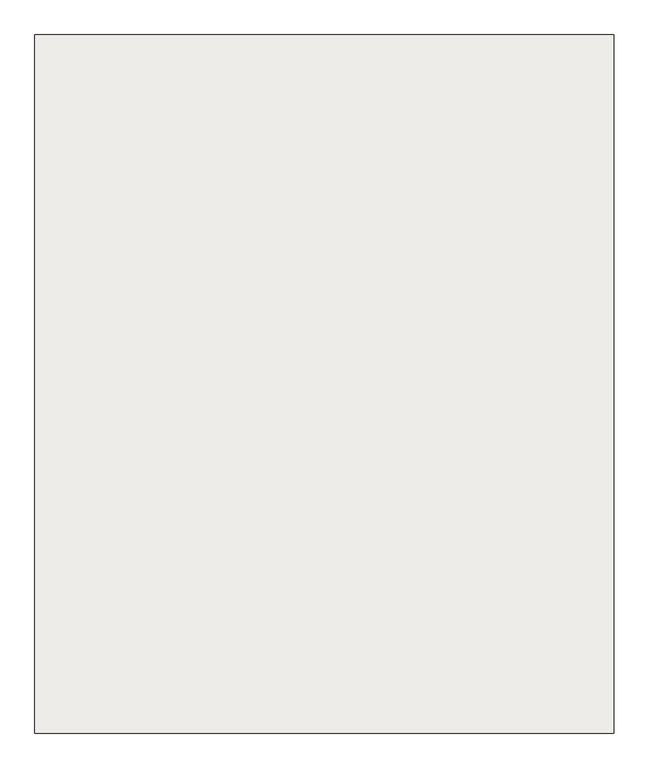
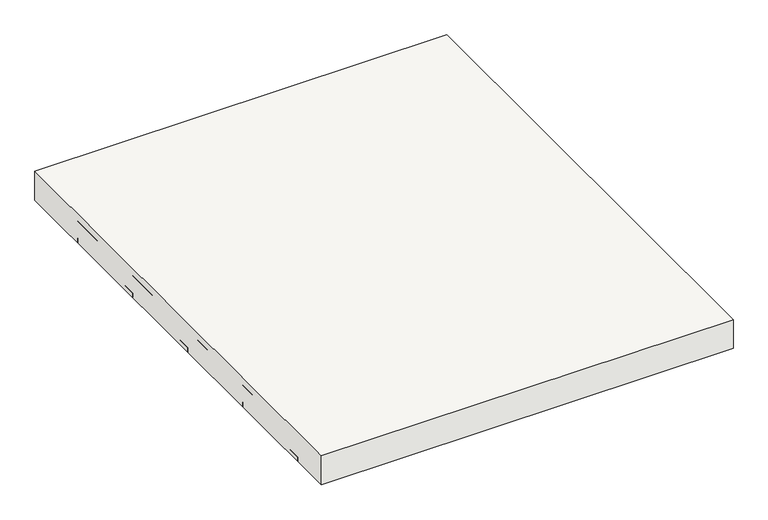
"""IFC4 building model written with IfcOpenShell, lengths in millimetres: slab geometry, Pano 13 (16 cm)."""

import ifcopenshell
import ifcopenshell.guid

model = None  # the IFC model being written
_history = None  # IfcOwnerHistory: only IFC2X3 demands one
_inside = {}  # id of a spatial element -> (the spatial element, [elements in it])
_under = {}  # id of a project, library or spatial element -> (it, [spatial elements below it])
_declared = {}  # id of a project -> (the project, [libraries it declares])
_typed = {}  # id of a type object -> (the type object, [elements of that type])
_made_of = {}  # id of a material, layer set ... -> (it, [elements and type objects made of it])


def new_model(schema):
    """Start an empty IFC model of exactly this schema.

    Asked for "IFC4X3", IfcOpenShell would pick the latest addendum, in which some entities
    have other attributes; the version numbers below select the first issue.
    IFC2X3 requires an IfcOwnerHistory on every rooted entity: one is made here for all.
    """
    global model, _history
    if schema == "IFC4X3":
        model = ifcopenshell.file(schema_version=(4, 3, 0, 0))
    else:
        model = ifcopenshell.file(schema=schema)
    _inside.clear()
    _under.clear()
    _declared.clear()
    _typed.clear()
    _made_of.clear()
    _history = None
    if model.schema == "IFC2X3":
        org = make("IfcOrganization", Name="unknown")
        user = make(
            "IfcPersonAndOrganization",
            ThePerson=make("IfcPerson", FamilyName="unknown"),
            TheOrganization=org,
        )
        app = make(
            "IfcApplication",
            ApplicationDeveloper=org,
            Version="unknown",
            ApplicationFullName="unknown",
            ApplicationIdentifier="unknown",
        )
        _history = make(
            "IfcOwnerHistory",
            OwningUser=user,
            OwningApplication=app,
            ChangeAction="ADDED",
            CreationDate=0,
        )
    return model


def make(cls, **values):
    """One entity of the class cls with the attributes given. An attribute that is None is left unset."""
    return model.create_entity(
        cls, **{name: value for name, value in values.items() if value is not None}
    )


def rooted(cls, **values):
    """An entity with a GlobalId (a new one), such as an element, a storey or a relation."""
    return make(cls, GlobalId=ifcopenshell.guid.new(), OwnerHistory=_history, **values)


def si_unit(unit_type, name, prefix=None):
    """IfcSIUnit, for example si_unit("LENGTHUNIT", "METRE", prefix="MILLI")."""
    return make("IfcSIUnit", UnitType=unit_type, Prefix=prefix, Name=name)


def assignment(units):
    """IfcUnitAssignment: the units of a project."""
    return None if units is None else make("IfcUnitAssignment", Units=units)


def point(xyz):
    """IfcCartesianPoint."""
    return None if xyz is None else make("IfcCartesianPoint", Coordinates=xyz)


def direction(xyz):
    """IfcDirection."""
    return None if xyz is None else make("IfcDirection", DirectionRatios=xyz)


def frame(location, z_axis=None, x_axis=None):
    """IfcAxis2Placement3D, a coordinate frame: its origin and axes. An axis left out is left unset."""
    return make(
        "IfcAxis2Placement3D",
        Location=point(location),
        Axis=direction(z_axis),
        RefDirection=direction(x_axis),
    )


def origin():
    """The frame at (0, 0, 0) with its axes left unset."""
    return frame((0.0, 0.0, 0.0))


def origin_with_axes():
    """The frame at (0, 0, 0) with the z axis (0, 0, 1) and the x axis (1, 0, 0) written out."""
    return frame((0.0, 0.0, 0.0), z_axis=(0.0, 0.0, 1.0), x_axis=(1.0, 0.0, 0.0))


def place(relative_to, where):
    """IfcLocalPlacement: puts the frame where relative to a parent placement (None: the world)."""
    return make(
        "IfcLocalPlacement", PlacementRelTo=relative_to, RelativePlacement=where
    )


def context(
    kind, dimensions, precision=None, world=None, true_north=None, identifier=None
):
    """IfcGeometricRepresentationContext, for example the 3D "Model" context."""
    return make(
        "IfcGeometricRepresentationContext",
        ContextIdentifier=identifier,
        ContextType=kind,
        CoordinateSpaceDimension=dimensions,
        Precision=precision,
        WorldCoordinateSystem=world,
        TrueNorth=true_north,
    )


def project(units=None, contexts=None):
    """IfcProject with its units and contexts."""
    return rooted(
        "IfcProject",
        Name="project",
        RepresentationContexts=contexts,
        UnitsInContext=assignment(units),
    )


def spatial(cls, under=None, at=None, **own):
    """A site, building, storey or space (cls), placed at a placement, below another one or the project."""
    s = rooted(cls, ObjectPlacement=at, **own)
    if under is not None:
        _under.setdefault(under.id(), (under, []))[1].append(s)
    return s


def polyline(points):
    """IfcPolyline through the points."""
    return make("IfcPolyline", Points=[point(p) for p in points])


def outline(outer, holes=None, kind="AREA"):
    """IfcArbitraryClosedProfileDef: a profile drawn as a closed curve; with holes, ...WithVoids."""
    if holes is None:
        return make("IfcArbitraryClosedProfileDef", ProfileType=kind, OuterCurve=outer)
    return make(
        "IfcArbitraryProfileDefWithVoids",
        ProfileType=kind,
        OuterCurve=outer,
        InnerCurves=holes,
    )


def extrude(swept, where, along, depth):
    """IfcExtrudedAreaSolid: the profile swept, set in the frame where, extruded along a direction by depth."""
    return make(
        "IfcExtrudedAreaSolid",
        SweptArea=swept,
        Position=where,
        ExtrudedDirection=direction(along),
        Depth=depth,
    )


def shape(context_of_items, identifier, shape_type, items):
    """IfcShapeRepresentation: the items that make up one representation, for example the "Body"."""
    return make(
        "IfcShapeRepresentation",
        ContextOfItems=context_of_items,
        RepresentationIdentifier=identifier,
        RepresentationType=shape_type,
        Items=items,
    )


def source(mapping_origin, context_of_items, identifier, shape_type, items):
    """IfcRepresentationMap: a shape defined once, which mapped items show again and again."""
    return make(
        "IfcRepresentationMap",
        MappingOrigin=mapping_origin,
        MappedRepresentation=shape(context_of_items, identifier, shape_type, items),
    )


def transform(
    local_origin,
    x_axis=None,
    y_axis=None,
    z_axis=None,
    scale=None,
    scale2=None,
    scale3=None,
    uniform=True,
):
    """IfcCartesianTransformationOperator3D, or its non-uniform kind. x_axis, y_axis, z_axis: its Axis1, 2, 3."""
    if uniform:
        return make(
            "IfcCartesianTransformationOperator3D",
            Axis1=direction(x_axis),
            Axis2=direction(y_axis),
            LocalOrigin=point(local_origin),
            Scale=scale,
            Axis3=direction(z_axis),
        )
    return make(
        "IfcCartesianTransformationOperator3DnonUniform",
        Axis1=direction(x_axis),
        Axis2=direction(y_axis),
        LocalOrigin=point(local_origin),
        Scale=scale,
        Axis3=direction(z_axis),
        Scale2=scale2,
        Scale3=scale3,
    )


def mapped(mapping_source, mapping_target):
    """IfcMappedItem: shows the shape of a source again, moved by a transform."""
    return make(
        "IfcMappedItem", MappingSource=mapping_source, MappingTarget=mapping_target
    )


def made_of(thing, what):
    """Note that an element or type object is made of a material, layer set ...; save() writes the relation."""
    if what is not None:
        _made_of.setdefault(what.id(), (what, []))[1].append(thing)
    return thing


def element(
    cls,
    number,
    at=None,
    inside=None,
    cuts=None,
    type_object=None,
    material=None,
    context=None,
    identifier="Body",
    shape_type=None,
    held_by="IfcProductDefinitionShape",
    body=None,
    shapes=None,
    **own,
):
    """One element of the class cls, such as IfcWall. Its Tag is "e" and its number.

    at: its placement. inside: the storey or other place that contains it. cuts: it is an
    opening in that element (IfcRelVoidsElement). A single representation is given by context,
    identifier, shape_type and body (its items); several are given by shapes. held_by: the class
    of the entity that holds the representations. save() writes the other relations.
    """
    e = rooted(cls, Tag="e%d" % number, ObjectPlacement=at, **own)
    if body is not None:
        shapes = [shape(context, identifier, shape_type, body)]
    if shapes is not None:
        e.Representation = make(held_by, Representations=shapes)
    if inside is not None:
        _inside.setdefault(inside.id(), (inside, []))[1].append(e)
    if cuts is not None:
        rooted(
            "IfcRelVoidsElement", RelatingBuildingElement=cuts, RelatedOpeningElement=e
        )
    if type_object is not None:
        _typed.setdefault(type_object.id(), (type_object, []))[1].append(e)
    return made_of(e, material)


def aggregate(whole, parts):
    """IfcRelAggregates: a whole, such as a stair, and the parts it consists of."""
    return rooted("IfcRelAggregates", RelatingObject=whole, RelatedObjects=parts)


def save(model, path):
    """Write the relations noted so far, then the file.

    IfcRelAggregates (storeys below a building ...), IfcRelContainedInSpatialStructure (elements
    in a storey), IfcRelDefinesByType, IfcRelAssociatesMaterial and IfcRelDeclares: one each for
    every whole, place, type object, material and project.
    """
    for whole, parts in _under.values():
        aggregate(whole, parts)
    for where, things in _inside.values():
        rooted(
            "IfcRelContainedInSpatialStructure",
            RelatedElements=things,
            RelatingStructure=where,
        )
    for kind, things in _typed.values():
        rooted("IfcRelDefinesByType", RelatedObjects=things, RelatingType=kind)
    for what, things in _made_of.values():
        rooted("IfcRelAssociatesMaterial", RelatedObjects=things, RelatingMaterial=what)
    for by, libraries in _declared.values():
        rooted("IfcRelDeclares", RelatingContext=by, RelatedDefinitions=libraries)
    model.write(path)


def slab_75a4034b(model_context):
    return source(origin(), model_context, "Body", "SweptSolid", [
        extrude(outline(polyline([(2395.00107, 8095.0), (4555.0, 8095.0), (4555.0, 5490.0), (2395.00107, 5490.0), (2395.00107, 8095.0)])), origin_with_axes(), (0.0, 0.0, 1.0), 160.0),
        extrude(outline(polyline([(2395.00107, 7204.0), (2395.00107, 7344.0), (4555.0, 7344.0), (4555.0, 7204.0), (2395.00107, 7204.0)])), origin_with_axes(), (0.0, 0.0, 1.0), 24.0),
        extrude(outline(polyline([(3895.00107, 6844.0), (3895.00107, 7204.0), (4390.00107, 7204.0), (4390.00107, 6844.0), (3895.00107, 6844.0)])), origin_with_axes(), (0.0, 0.0, 1.0), 120.0),
        extrude(outline(polyline([(3895.00107, 5844.0), (3895.00107, 6204.0), (4390.00107, 6204.0), (4390.00107, 5844.0), (3895.00107, 5844.0)])), origin_with_axes(), (0.0, 0.0, 1.0), 120.0),
        extrude(outline(polyline([(2395.00107, 6344.0), (2395.00107, 6704.0), (2890.00107, 6704.0), (2890.00107, 6344.0), (2395.00107, 6344.0)])), origin_with_axes(), (0.0, 0.0, 1.0), 120.0),
        extrude(outline(polyline([(2395.00107, 6204.0), (2395.00107, 6344.0), (4555.0, 6344.0), (4555.0, 6204.0), (2395.00107, 6204.0)])), origin_with_axes(), (0.0, 0.0, 1.0), 24.0),
        extrude(outline(polyline([(3395.00107, 6844.0), (3395.00107, 7204.0), (3890.00107, 7204.0), (3890.00107, 6844.0), (3395.00107, 6844.0)])), origin_with_axes(), (0.0, 0.0, 1.0), 120.0),
        extrude(outline(polyline([(4395.00107, 5844.0), (4395.00107, 6204.0), (4550.0, 6204.0), (4550.0, 5844.0), (4395.00107, 5844.0)])), origin_with_axes(), (0.0, 0.0, 1.0), 120.0),
        extrude(outline(polyline([(4395.00107, 6844.0), (4395.00107, 7204.0), (4550.0, 7204.0), (4550.0, 6844.0), (4395.00107, 6844.0)])), origin_with_axes(), (0.0, 0.0, 1.0), 120.0),
        extrude(outline(polyline([(2895.00107, 5844.0), (2895.00107, 6204.0), (3390.00107, 6204.0), (3390.00107, 5844.0), (2895.00107, 5844.0)])), origin_with_axes(), (0.0, 0.0, 1.0), 120.0),
        extrude(outline(polyline([(2895.00107, 7344.0), (2895.00107, 7704.0), (3390.00107, 7704.0), (3390.00107, 7344.0), (2895.00107, 7344.0)])), origin_with_axes(), (0.0, 0.0, 1.0), 120.0),
        extrude(outline(polyline([(2395.00107, 6844.0), (2395.00107, 7204.0), (2890.00107, 7204.0), (2890.00107, 6844.0), (2395.00107, 6844.0)])), origin_with_axes(), (0.0, 0.0, 1.0), 120.0),
        extrude(outline(polyline([(2395.00107, 7704.0), (2395.00107, 7844.0), (4555.0, 7844.0), (4555.0, 7704.0), (2395.00107, 7704.0)])), origin_with_axes(), (0.0, 0.0, 1.0), 24.0),
        extrude(outline(polyline([(3395.00107, 7344.0), (3395.00107, 7704.0), (3890.00107, 7704.0), (3890.00107, 7344.0), (3395.00107, 7344.0)])), origin_with_axes(), (0.0, 0.0, 1.0), 120.0),
        extrude(outline(polyline([(2395.00107, 6704.0), (2395.00107, 6844.0), (4555.0, 6844.0), (4555.0, 6704.0), (2395.00107, 6704.0)])), origin_with_axes(), (0.0, 0.0, 1.0), 24.0),
        extrude(outline(polyline([(2895.00107, 6344.0), (2895.00107, 6704.0), (3390.00107, 6704.0), (3390.00107, 6344.0), (2895.00107, 6344.0)])), origin_with_axes(), (0.0, 0.0, 1.0), 120.0),
        extrude(outline(polyline([(2395.00107, 5844.0), (2395.00107, 6204.0), (2890.00107, 6204.0), (2890.00107, 5844.0), (2395.00107, 5844.0)])), origin_with_axes(), (0.0, 0.0, 1.0), 120.0),
        extrude(outline(polyline([(4395.00107, 7344.0), (4395.00107, 7704.0), (4550.0, 7704.0), (4550.0, 7344.0), (4395.00107, 7344.0)])), origin_with_axes(), (0.0, 0.0, 1.0), 120.0),
        extrude(outline(polyline([(3395.00107, 6344.0), (3395.00107, 6704.0), (3890.00107, 6704.0), (3890.00107, 6344.0), (3395.00107, 6344.0)])), origin_with_axes(), (0.0, 0.0, 1.0), 120.0),
        extrude(outline(polyline([(2395.00107, 5704.0), (2395.00107, 5844.0), (4555.0, 5844.0), (4555.0, 5704.0), (2395.00107, 5704.0)])), origin_with_axes(), (0.0, 0.0, 1.0), 24.0),
        extrude(outline(polyline([(2395.00107, 7344.0), (2395.00107, 7704.0), (2890.00107, 7704.0), (2890.00107, 7344.0), (2395.00107, 7344.0)])), origin_with_axes(), (0.0, 0.0, 1.0), 120.0),
        extrude(outline(polyline([(3895.00107, 6344.0), (3895.00107, 6704.0), (4390.00107, 6704.0), (4390.00107, 6344.0), (3895.00107, 6344.0)])), origin_with_axes(), (0.0, 0.0, 1.0), 120.0),
        extrude(outline(polyline([(3895.00107, 7344.0), (3895.00107, 7704.0), (4390.00107, 7704.0), (4390.00107, 7344.0), (3895.00107, 7344.0)])), origin_with_axes(), (0.0, 0.0, 1.0), 120.0),
        extrude(outline(polyline([(2895.00107, 6844.0), (2895.00107, 7204.0), (3390.00107, 7204.0), (3390.00107, 6844.0), (2895.00107, 6844.0)])), origin_with_axes(), (0.0, 0.0, 1.0), 120.0),
        extrude(outline(polyline([(3395.00107, 5844.0), (3395.00107, 6204.0), (3890.00107, 6204.0), (3890.00107, 5844.0), (3395.00107, 5844.0)])), origin_with_axes(), (0.0, 0.0, 1.0), 120.0),
        extrude(outline(polyline([(4395.00107, 6344.0), (4395.00107, 6704.0), (4550.0, 6704.0), (4550.0, 6344.0), (4395.00107, 6344.0)])), origin_with_axes(), (0.0, 0.0, 1.0), 120.0),
    ])


if __name__ == "__main__":
    model = new_model("IFC4")
    model_context = context("Model", 3, world=origin())
    ifc_project = project(units=[si_unit("LENGTHUNIT", "METRE", prefix="MILLI")], contexts=[model_context])
    site = spatial("IfcSite", under=ifc_project)
    building = spatial("IfcBuilding", under=site)
    placement = place(None, origin())
    slab_shape = slab_75a4034b(model_context)
    element("IfcSlab", 1, ObjectType="Pano 13 (16 cm)", at=placement, inside=building, context=model_context, shape_type="MappedRepresentation", body=[
        mapped(slab_shape, transform((0.0, 0.0, 0.0), x_axis=(1.0, 0.0, 0.0), y_axis=(0.0, 1.0, 0.0), z_axis=(0.0, 0.0, 1.0))),
    ])
    save(model, "model.ifc")

# Revit data of these elements
# Element 1 (IfcSlab, "Pano 13 (16 cm)")
#   Materials on its faces: "Molde de poliestireno", "Concreto armado", "RGB 168-169-158"
# Materials
#   "Molde de poliestireno": class "Não atribuído", colour RGB 255 255 255, transparency 0
#   "Concreto armado": class "Não atribuído", colour RGB 168 169 158, transparency 0
#   "RGB 168-169-158": class "Não atribuído", colour RGB 168 169 158, transparency 0
